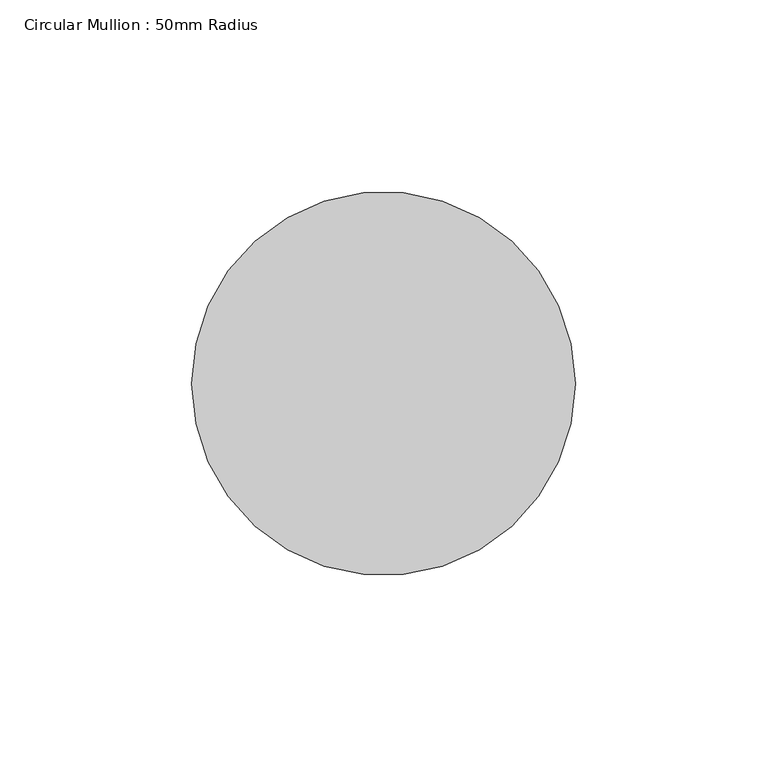
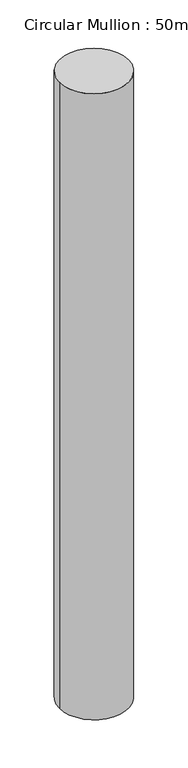
"""IFC4 building model written with IfcOpenShell, lengths in millimetres: member geometry, Circular Mullion : 50mm Radius."""

import ifcopenshell
import ifcopenshell.guid

model = None  # the IFC model being written
_history = None  # IfcOwnerHistory: only IFC2X3 demands one
_inside = {}  # id of a spatial element -> (the spatial element, [elements in it])
_under = {}  # id of a project, library or spatial element -> (it, [spatial elements below it])
_declared = {}  # id of a project -> (the project, [libraries it declares])
_typed = {}  # id of a type object -> (the type object, [elements of that type])
_made_of = {}  # id of a material, layer set ... -> (it, [elements and type objects made of it])


def new_model(schema):
    """Start an empty IFC model of exactly this schema.

    Asked for "IFC4X3", IfcOpenShell would pick the latest addendum, in which some entities
    have other attributes; the version numbers below select the first issue.
    IFC2X3 requires an IfcOwnerHistory on every rooted entity: one is made here for all.
    """
    global model, _history
    if schema == "IFC4X3":
        model = ifcopenshell.file(schema_version=(4, 3, 0, 0))
    else:
        model = ifcopenshell.file(schema=schema)
    _inside.clear()
    _under.clear()
    _declared.clear()
    _typed.clear()
    _made_of.clear()
    _history = None
    if model.schema == "IFC2X3":
        org = make("IfcOrganization", Name="unknown")
        user = make(
            "IfcPersonAndOrganization",
            ThePerson=make("IfcPerson", FamilyName="unknown"),
            TheOrganization=org,
        )
        app = make(
            "IfcApplication",
            ApplicationDeveloper=org,
            Version="unknown",
            ApplicationFullName="unknown",
            ApplicationIdentifier="unknown",
        )
        _history = make(
            "IfcOwnerHistory",
            OwningUser=user,
            OwningApplication=app,
            ChangeAction="ADDED",
            CreationDate=0,
        )
    return model


def make(cls, **values):
    """One entity of the class cls with the attributes given. An attribute that is None is left unset."""
    return model.create_entity(
        cls, **{name: value for name, value in values.items() if value is not None}
    )


def rooted(cls, **values):
    """An entity with a GlobalId (a new one), such as an element, a storey or a relation."""
    return make(cls, GlobalId=ifcopenshell.guid.new(), OwnerHistory=_history, **values)


def si_unit(unit_type, name, prefix=None):
    """IfcSIUnit, for example si_unit("LENGTHUNIT", "METRE", prefix="MILLI")."""
    return make("IfcSIUnit", UnitType=unit_type, Prefix=prefix, Name=name)


def assignment(units):
    """IfcUnitAssignment: the units of a project."""
    return None if units is None else make("IfcUnitAssignment", Units=units)


def point(xyz):
    """IfcCartesianPoint."""
    return None if xyz is None else make("IfcCartesianPoint", Coordinates=xyz)


def direction(xyz):
    """IfcDirection."""
    return None if xyz is None else make("IfcDirection", DirectionRatios=xyz)


def frame(location, z_axis=None, x_axis=None):
    """IfcAxis2Placement3D, a coordinate frame: its origin and axes. An axis left out is left unset."""
    return make(
        "IfcAxis2Placement3D",
        Location=point(location),
        Axis=direction(z_axis),
        RefDirection=direction(x_axis),
    )


def frame_2d(location, x_axis=None):
    """IfcAxis2Placement2D, a coordinate frame in the plane: its origin and x axis."""
    return make(
        "IfcAxis2Placement2D", Location=point(location), RefDirection=direction(x_axis)
    )


def origin():
    """The frame at (0, 0, 0) with its axes left unset."""
    return frame((0.0, 0.0, 0.0))


def origin_2d():
    """The frame at (0, 0) in the plane with its x axis left unset."""
    return frame_2d((0.0, 0.0))


def place(relative_to, where):
    """IfcLocalPlacement: puts the frame where relative to a parent placement (None: the world)."""
    return make(
        "IfcLocalPlacement", PlacementRelTo=relative_to, RelativePlacement=where
    )


def context(
    kind, dimensions, precision=None, world=None, true_north=None, identifier=None
):
    """IfcGeometricRepresentationContext, for example the 3D "Model" context."""
    return make(
        "IfcGeometricRepresentationContext",
        ContextIdentifier=identifier,
        ContextType=kind,
        CoordinateSpaceDimension=dimensions,
        Precision=precision,
        WorldCoordinateSystem=world,
        TrueNorth=true_north,
    )


def project(units=None, contexts=None):
    """IfcProject with its units and contexts."""
    return rooted(
        "IfcProject",
        Name="project",
        RepresentationContexts=contexts,
        UnitsInContext=assignment(units),
    )


def spatial(cls, under=None, at=None, **own):
    """A site, building, storey or space (cls), placed at a placement, below another one or the project."""
    s = rooted(cls, ObjectPlacement=at, **own)
    if under is not None:
        _under.setdefault(under.id(), (under, []))[1].append(s)
    return s


def circle_curve(where, radius):
    """IfcCircle in the frame where."""
    return make("IfcCircle", Position=where, Radius=radius)


def trimmed(basis, trim1, trim2, sense, master):
    """IfcTrimmedCurve: the piece of a basis curve between two trims."""
    return make(
        "IfcTrimmedCurve",
        BasisCurve=basis,
        Trim1=trim1,
        Trim2=trim2,
        SenseAgreement=sense,
        MasterRepresentation=master,
    )


def segment(curve, same_sense, transition):
    """IfcCompositeCurveSegment."""
    return make(
        "IfcCompositeCurveSegment",
        Transition=transition,
        SameSense=same_sense,
        ParentCurve=curve,
    )


def composite_curve(segments, self_intersect=None):
    """IfcCompositeCurve: segments joined end to end."""
    return make("IfcCompositeCurve", Segments=segments, SelfIntersect=self_intersect)


def outline(outer, holes=None, kind="AREA"):
    """IfcArbitraryClosedProfileDef: a profile drawn as a closed curve; with holes, ...WithVoids."""
    if holes is None:
        return make("IfcArbitraryClosedProfileDef", ProfileType=kind, OuterCurve=outer)
    return make(
        "IfcArbitraryProfileDefWithVoids",
        ProfileType=kind,
        OuterCurve=outer,
        InnerCurves=holes,
    )


def extrude(swept, where, along, depth):
    """IfcExtrudedAreaSolid: the profile swept, set in the frame where, extruded along a direction by depth."""
    return make(
        "IfcExtrudedAreaSolid",
        SweptArea=swept,
        Position=where,
        ExtrudedDirection=direction(along),
        Depth=depth,
    )


def shape(context_of_items, identifier, shape_type, items):
    """IfcShapeRepresentation: the items that make up one representation, for example the "Body"."""
    return make(
        "IfcShapeRepresentation",
        ContextOfItems=context_of_items,
        RepresentationIdentifier=identifier,
        RepresentationType=shape_type,
        Items=items,
    )


def source(mapping_origin, context_of_items, identifier, shape_type, items):
    """IfcRepresentationMap: a shape defined once, which mapped items show again and again."""
    return make(
        "IfcRepresentationMap",
        MappingOrigin=mapping_origin,
        MappedRepresentation=shape(context_of_items, identifier, shape_type, items),
    )


def transform(
    local_origin,
    x_axis=None,
    y_axis=None,
    z_axis=None,
    scale=None,
    scale2=None,
    scale3=None,
    uniform=True,
):
    """IfcCartesianTransformationOperator3D, or its non-uniform kind. x_axis, y_axis, z_axis: its Axis1, 2, 3."""
    if uniform:
        return make(
            "IfcCartesianTransformationOperator3D",
            Axis1=direction(x_axis),
            Axis2=direction(y_axis),
            LocalOrigin=point(local_origin),
            Scale=scale,
            Axis3=direction(z_axis),
        )
    return make(
        "IfcCartesianTransformationOperator3DnonUniform",
        Axis1=direction(x_axis),
        Axis2=direction(y_axis),
        LocalOrigin=point(local_origin),
        Scale=scale,
        Axis3=direction(z_axis),
        Scale2=scale2,
        Scale3=scale3,
    )


def mapped(mapping_source, mapping_target):
    """IfcMappedItem: shows the shape of a source again, moved by a transform."""
    return make(
        "IfcMappedItem", MappingSource=mapping_source, MappingTarget=mapping_target
    )


def made_of(thing, what):
    """Note that an element or type object is made of a material, layer set ...; save() writes the relation."""
    if what is not None:
        _made_of.setdefault(what.id(), (what, []))[1].append(thing)
    return thing


def element(
    cls,
    number,
    at=None,
    inside=None,
    cuts=None,
    type_object=None,
    material=None,
    context=None,
    identifier="Body",
    shape_type=None,
    held_by="IfcProductDefinitionShape",
    body=None,
    shapes=None,
    **own,
):
    """One element of the class cls, such as IfcWall. Its Tag is "e" and its number.

    at: its placement. inside: the storey or other place that contains it. cuts: it is an
    opening in that element (IfcRelVoidsElement). A single representation is given by context,
    identifier, shape_type and body (its items); several are given by shapes. held_by: the class
    of the entity that holds the representations. save() writes the other relations.
    """
    e = rooted(cls, Tag="e%d" % number, ObjectPlacement=at, **own)
    if body is not None:
        shapes = [shape(context, identifier, shape_type, body)]
    if shapes is not None:
        e.Representation = make(held_by, Representations=shapes)
    if inside is not None:
        _inside.setdefault(inside.id(), (inside, []))[1].append(e)
    if cuts is not None:
        rooted(
            "IfcRelVoidsElement", RelatingBuildingElement=cuts, RelatedOpeningElement=e
        )
    if type_object is not None:
        _typed.setdefault(type_object.id(), (type_object, []))[1].append(e)
    return made_of(e, material)


def aggregate(whole, parts):
    """IfcRelAggregates: a whole, such as a stair, and the parts it consists of."""
    return rooted("IfcRelAggregates", RelatingObject=whole, RelatedObjects=parts)


def save(model, path):
    """Write the relations noted so far, then the file.

    IfcRelAggregates (storeys below a building ...), IfcRelContainedInSpatialStructure (elements
    in a storey), IfcRelDefinesByType, IfcRelAssociatesMaterial and IfcRelDeclares: one each for
    every whole, place, type object, material and project.
    """
    for whole, parts in _under.values():
        aggregate(whole, parts)
    for where, things in _inside.values():
        rooted(
            "IfcRelContainedInSpatialStructure",
            RelatedElements=things,
            RelatingStructure=where,
        )
    for kind, things in _typed.values():
        rooted("IfcRelDefinesByType", RelatedObjects=things, RelatingType=kind)
    for what, things in _made_of.values():
        rooted("IfcRelAssociatesMaterial", RelatedObjects=things, RelatingMaterial=what)
    for by, libraries in _declared.values():
        rooted("IfcRelDeclares", RelatingContext=by, RelatedDefinitions=libraries)
    model.write(path)


def circular_mullion_50mm_radius_36e3f533(model_context):
    return source(origin(), model_context, "Body", "SweptSolid", [
        extrude(outline(composite_curve([segment(trimmed(circle_curve(origin_2d(), 50.0), [point((50.0, 0.0))], [point((-50.0, 0.0))], False, "CARTESIAN"), True, "CONTINUOUS"), segment(trimmed(circle_curve(origin_2d(), 50.0), [point((-50.0, 0.0))], [point((50.0, 0.0))], False, "CARTESIAN"), True, "CONTINUOUS")], self_intersect=False)), frame((0.0, 0.0, -959.817448), z_axis=(0.0, 0.0, 1.0), x_axis=(1.0, 0.0, 0.0)), (0.0, 0.0, 1.0), 959.817448),
    ])


if __name__ == "__main__":
    model = new_model("IFC4")
    model_context = context("Model", 3, world=origin())
    ifc_project = project(units=[si_unit("LENGTHUNIT", "METRE", prefix="MILLI")], contexts=[model_context])
    site = spatial("IfcSite", under=ifc_project)
    building = spatial("IfcBuilding", under=site)
    placement = place(None, origin())
    circular_mullion_50mm_radius_shape = circular_mullion_50mm_radius_36e3f533(model_context)
    element("IfcMember", 1, ObjectType="Circular Mullion : 50mm Radius", at=placement, inside=building, context=model_context, shape_type="MappedRepresentation", body=[
        mapped(circular_mullion_50mm_radius_shape, transform((0.0, 0.0, 0.0), x_axis=(1.0, 0.0, 0.0), y_axis=(0.0, 1.0, 0.0), z_axis=(0.0, 0.0, 1.0))),
    ])
    save(model, "model.ifc")

# Revit data of these elements
# Type "Circular Mullion : 50mm Radius"
#   built-in parameter 1007350 = 0.164042 (stored number, unit not read)
# Element 1 (IfcMember, "Circular Mullion : 50mm Radius")
#   Materials on its faces: "Aluminium"
# Materials
#   "Aluminium": class "Metal", colour RGB 247 247 247, transparency 0, Description = "Aluminium 6061", Cost = 0
